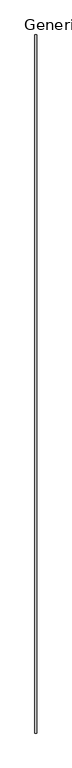
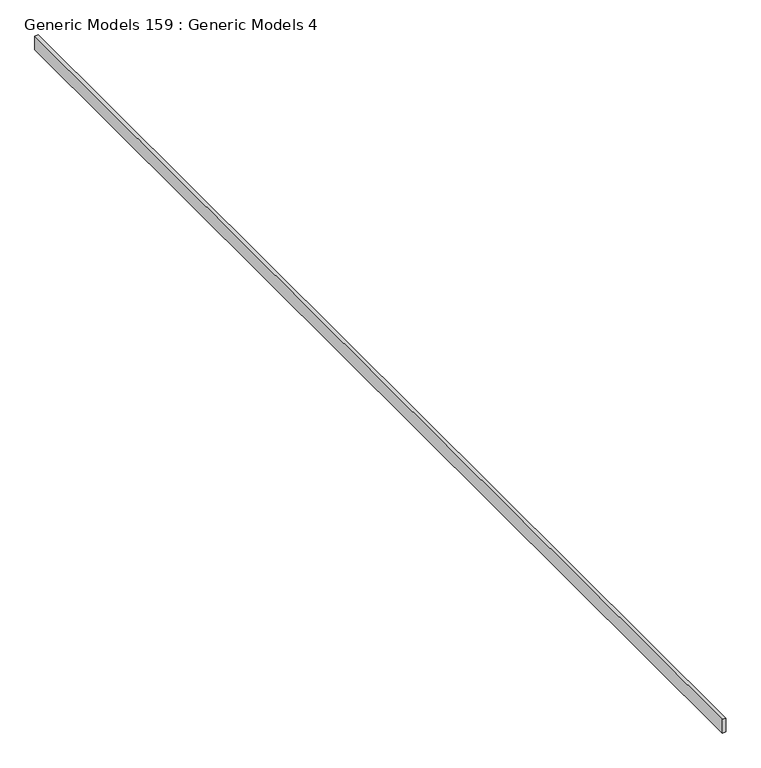
"""IFC4 building model written with IfcOpenShell, lengths in millimetres: proxy geometry, Generic Models 159 : Generic Models 4."""

import ifcopenshell
import ifcopenshell.guid

model = None  # the IFC model being written
_history = None  # IfcOwnerHistory: only IFC2X3 demands one
_inside = {}  # id of a spatial element -> (the spatial element, [elements in it])
_under = {}  # id of a project, library or spatial element -> (it, [spatial elements below it])
_declared = {}  # id of a project -> (the project, [libraries it declares])
_typed = {}  # id of a type object -> (the type object, [elements of that type])
_made_of = {}  # id of a material, layer set ... -> (it, [elements and type objects made of it])


def new_model(schema):
    """Start an empty IFC model of exactly this schema.

    Asked for "IFC4X3", IfcOpenShell would pick the latest addendum, in which some entities
    have other attributes; the version numbers below select the first issue.
    IFC2X3 requires an IfcOwnerHistory on every rooted entity: one is made here for all.
    """
    global model, _history
    if schema == "IFC4X3":
        model = ifcopenshell.file(schema_version=(4, 3, 0, 0))
    else:
        model = ifcopenshell.file(schema=schema)
    _inside.clear()
    _under.clear()
    _declared.clear()
    _typed.clear()
    _made_of.clear()
    _history = None
    if model.schema == "IFC2X3":
        org = make("IfcOrganization", Name="unknown")
        user = make(
            "IfcPersonAndOrganization",
            ThePerson=make("IfcPerson", FamilyName="unknown"),
            TheOrganization=org,
        )
        app = make(
            "IfcApplication",
            ApplicationDeveloper=org,
            Version="unknown",
            ApplicationFullName="unknown",
            ApplicationIdentifier="unknown",
        )
        _history = make(
            "IfcOwnerHistory",
            OwningUser=user,
            OwningApplication=app,
            ChangeAction="ADDED",
            CreationDate=0,
        )
    return model


def make(cls, **values):
    """One entity of the class cls with the attributes given. An attribute that is None is left unset."""
    return model.create_entity(
        cls, **{name: value for name, value in values.items() if value is not None}
    )


def rooted(cls, **values):
    """An entity with a GlobalId (a new one), such as an element, a storey or a relation."""
    return make(cls, GlobalId=ifcopenshell.guid.new(), OwnerHistory=_history, **values)


def si_unit(unit_type, name, prefix=None):
    """IfcSIUnit, for example si_unit("LENGTHUNIT", "METRE", prefix="MILLI")."""
    return make("IfcSIUnit", UnitType=unit_type, Prefix=prefix, Name=name)


def assignment(units):
    """IfcUnitAssignment: the units of a project."""
    return None if units is None else make("IfcUnitAssignment", Units=units)


def point(xyz):
    """IfcCartesianPoint."""
    return None if xyz is None else make("IfcCartesianPoint", Coordinates=xyz)


def direction(xyz):
    """IfcDirection."""
    return None if xyz is None else make("IfcDirection", DirectionRatios=xyz)


def frame(location, z_axis=None, x_axis=None):
    """IfcAxis2Placement3D, a coordinate frame: its origin and axes. An axis left out is left unset."""
    return make(
        "IfcAxis2Placement3D",
        Location=point(location),
        Axis=direction(z_axis),
        RefDirection=direction(x_axis),
    )


def origin():
    """The frame at (0, 0, 0) with its axes left unset."""
    return frame((0.0, 0.0, 0.0))


def place(relative_to, where):
    """IfcLocalPlacement: puts the frame where relative to a parent placement (None: the world)."""
    return make(
        "IfcLocalPlacement", PlacementRelTo=relative_to, RelativePlacement=where
    )


def context(
    kind, dimensions, precision=None, world=None, true_north=None, identifier=None
):
    """IfcGeometricRepresentationContext, for example the 3D "Model" context."""
    return make(
        "IfcGeometricRepresentationContext",
        ContextIdentifier=identifier,
        ContextType=kind,
        CoordinateSpaceDimension=dimensions,
        Precision=precision,
        WorldCoordinateSystem=world,
        TrueNorth=true_north,
    )


def project(units=None, contexts=None):
    """IfcProject with its units and contexts."""
    return rooted(
        "IfcProject",
        Name="project",
        RepresentationContexts=contexts,
        UnitsInContext=assignment(units),
    )


def spatial(cls, under=None, at=None, **own):
    """A site, building, storey or space (cls), placed at a placement, below another one or the project."""
    s = rooted(cls, ObjectPlacement=at, **own)
    if under is not None:
        _under.setdefault(under.id(), (under, []))[1].append(s)
    return s


def polyline(points):
    """IfcPolyline through the points."""
    return make("IfcPolyline", Points=[point(p) for p in points])


def outline(outer, holes=None, kind="AREA"):
    """IfcArbitraryClosedProfileDef: a profile drawn as a closed curve; with holes, ...WithVoids."""
    if holes is None:
        return make("IfcArbitraryClosedProfileDef", ProfileType=kind, OuterCurve=outer)
    return make(
        "IfcArbitraryProfileDefWithVoids",
        ProfileType=kind,
        OuterCurve=outer,
        InnerCurves=holes,
    )


def extrude(swept, where, along, depth):
    """IfcExtrudedAreaSolid: the profile swept, set in the frame where, extruded along a direction by depth."""
    return make(
        "IfcExtrudedAreaSolid",
        SweptArea=swept,
        Position=where,
        ExtrudedDirection=direction(along),
        Depth=depth,
    )


def shape(context_of_items, identifier, shape_type, items):
    """IfcShapeRepresentation: the items that make up one representation, for example the "Body"."""
    return make(
        "IfcShapeRepresentation",
        ContextOfItems=context_of_items,
        RepresentationIdentifier=identifier,
        RepresentationType=shape_type,
        Items=items,
    )


def source(mapping_origin, context_of_items, identifier, shape_type, items):
    """IfcRepresentationMap: a shape defined once, which mapped items show again and again."""
    return make(
        "IfcRepresentationMap",
        MappingOrigin=mapping_origin,
        MappedRepresentation=shape(context_of_items, identifier, shape_type, items),
    )


def transform(
    local_origin,
    x_axis=None,
    y_axis=None,
    z_axis=None,
    scale=None,
    scale2=None,
    scale3=None,
    uniform=True,
):
    """IfcCartesianTransformationOperator3D, or its non-uniform kind. x_axis, y_axis, z_axis: its Axis1, 2, 3."""
    if uniform:
        return make(
            "IfcCartesianTransformationOperator3D",
            Axis1=direction(x_axis),
            Axis2=direction(y_axis),
            LocalOrigin=point(local_origin),
            Scale=scale,
            Axis3=direction(z_axis),
        )
    return make(
        "IfcCartesianTransformationOperator3DnonUniform",
        Axis1=direction(x_axis),
        Axis2=direction(y_axis),
        LocalOrigin=point(local_origin),
        Scale=scale,
        Axis3=direction(z_axis),
        Scale2=scale2,
        Scale3=scale3,
    )


def mapped(mapping_source, mapping_target):
    """IfcMappedItem: shows the shape of a source again, moved by a transform."""
    return make(
        "IfcMappedItem", MappingSource=mapping_source, MappingTarget=mapping_target
    )


def made_of(thing, what):
    """Note that an element or type object is made of a material, layer set ...; save() writes the relation."""
    if what is not None:
        _made_of.setdefault(what.id(), (what, []))[1].append(thing)
    return thing


def element(
    cls,
    number,
    at=None,
    inside=None,
    cuts=None,
    type_object=None,
    material=None,
    context=None,
    identifier="Body",
    shape_type=None,
    held_by="IfcProductDefinitionShape",
    body=None,
    shapes=None,
    **own,
):
    """One element of the class cls, such as IfcWall. Its Tag is "e" and its number.

    at: its placement. inside: the storey or other place that contains it. cuts: it is an
    opening in that element (IfcRelVoidsElement). A single representation is given by context,
    identifier, shape_type and body (its items); several are given by shapes. held_by: the class
    of the entity that holds the representations. save() writes the other relations.
    """
    e = rooted(cls, Tag="e%d" % number, ObjectPlacement=at, **own)
    if body is not None:
        shapes = [shape(context, identifier, shape_type, body)]
    if shapes is not None:
        e.Representation = make(held_by, Representations=shapes)
    if inside is not None:
        _inside.setdefault(inside.id(), (inside, []))[1].append(e)
    if cuts is not None:
        rooted(
            "IfcRelVoidsElement", RelatingBuildingElement=cuts, RelatedOpeningElement=e
        )
    if type_object is not None:
        _typed.setdefault(type_object.id(), (type_object, []))[1].append(e)
    return made_of(e, material)


def aggregate(whole, parts):
    """IfcRelAggregates: a whole, such as a stair, and the parts it consists of."""
    return rooted("IfcRelAggregates", RelatingObject=whole, RelatedObjects=parts)


def save(model, path):
    """Write the relations noted so far, then the file.

    IfcRelAggregates (storeys below a building ...), IfcRelContainedInSpatialStructure (elements
    in a storey), IfcRelDefinesByType, IfcRelAssociatesMaterial and IfcRelDeclares: one each for
    every whole, place, type object, material and project.
    """
    for whole, parts in _under.values():
        aggregate(whole, parts)
    for where, things in _inside.values():
        rooted(
            "IfcRelContainedInSpatialStructure",
            RelatedElements=things,
            RelatingStructure=where,
        )
    for kind, things in _typed.values():
        rooted("IfcRelDefinesByType", RelatedObjects=things, RelatingType=kind)
    for what, things in _made_of.values():
        rooted("IfcRelAssociatesMaterial", RelatedObjects=things, RelatingMaterial=what)
    for by, libraries in _declared.values():
        rooted("IfcRelDeclares", RelatingContext=by, RelatedDefinitions=libraries)
    model.write(path)


def generic_models_159_generic_models_4_a43d97e0(model_context):
    return source(origin(), model_context, "Body", "SweptSolid", [
        extrude(outline(polyline([(-10252.9339552, -5493.3230338), (-10290.0847239, -5493.3230338), (-10290.0847239, 7054.2769662), (-10252.9339552, 7054.2769662), (-10252.9339552, -5493.3230338)])), frame((0.0, 0.0, 122793.7234874), z_axis=(0.0, 0.0, 1.0), x_axis=(1.0, 0.0, 0.0)), (0.0, 0.0, 1.0), 152.4),
    ])


if __name__ == "__main__":
    model = new_model("IFC4")
    model_context = context("Model", 3, world=origin())
    ifc_project = project(units=[si_unit("LENGTHUNIT", "METRE", prefix="MILLI")], contexts=[model_context])
    site = spatial("IfcSite", under=ifc_project)
    building = spatial("IfcBuilding", under=site)
    placement = place(None, origin())
    generic_models_159_generic_models_4_shape = generic_models_159_generic_models_4_a43d97e0(model_context)
    element("IfcBuildingElementProxy", 1, Name="Generic Models 159 : Generic Models 4", ObjectType="Generic Models 159 : Generic Models 4", at=placement, inside=building, context=model_context, shape_type="MappedRepresentation", body=[
        mapped(generic_models_159_generic_models_4_shape, transform((0.0, 0.0, 0.0), x_axis=(1.0, 0.0, 0.0), y_axis=(0.0, 1.0, 0.0), z_axis=(0.0, 0.0, 1.0))),
    ])
    save(model, "model.ifc")

# Revit data of these elements
# Element 1 (IfcBuildingElementProxy, "Generic Models 159 : Generic Models 4")
#   Materials on its faces: "_SPLIT FACE STONE VENEER"
# Materials
#   "_SPLIT FACE STONE VENEER": class "Generic", colour RGB 125 135 145, transparency 0, Cost = 0
